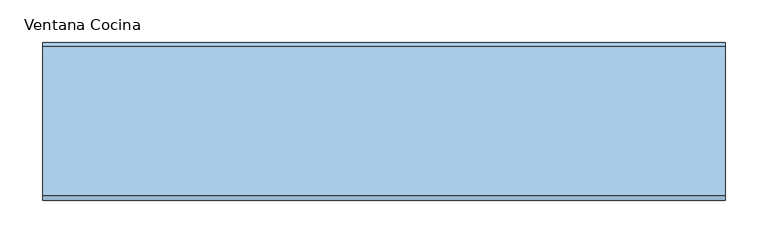
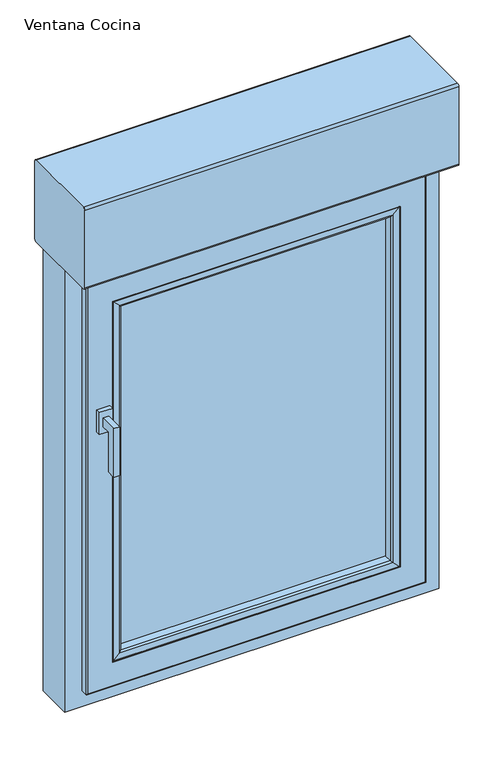
"""IFC4 building model written with IfcOpenShell, lengths in millimetres: window geometry, 2019_ES_Ventana_Replus_re80pvc301_10100_box_1-Hoja_con-Compacto : Ventana Cocina."""

from ifc_helpers import new_model, si_unit, point, frame, frame_2d, origin, place, context, project, spatial, polyline, circle_curve, ellipse_curve, trimmed, segment, composite_curve, outline, extrude, source, transform, mapped, element, save
from ifc_brep_helpers import plane_surface, cylinder_surface, advanced_brep


def ventana_cocina_c5497abf(model_context):
    return source(origin(), model_context, "Body", "SolidModel", [
        extrude(outline(composite_curve([segment(polyline([(55.0, 1810.0), (-120.0, 1810.0)]), True, "CONTINUOUS"), segment(trimmed(circle_curve(frame_2d((-120.0, 1815.0)), 5.0), [point((-120.0, 1810.0))], [point((-125.0, 1815.0))], False, "CARTESIAN"), True, "CONTINUOUS"), segment(polyline([(-125.0, 1815.0), (-125.0, 1990.0)]), True, "CONTINUOUS"), segment(trimmed(circle_curve(frame_2d((-120.0, 1990.0)), 5.0), [point((-125.0, 1990.0))], [point((-120.0, 1995.0))], False, "CARTESIAN"), True, "CONTINUOUS"), segment(polyline([(-120.0, 1995.0), (55.0, 1995.0)]), True, "CONTINUOUS"), segment(trimmed(circle_curve(frame_2d((55.0, 1990.0)), 5.0), [point((55.0, 1995.0))], [point((60.0, 1990.0))], False, "CARTESIAN"), True, "CONTINUOUS"), segment(polyline([(60.0, 1990.0), (60.0, 1815.0)]), True, "CONTINUOUS"), segment(trimmed(circle_curve(frame_2d((55.0, 1815.0)), 5.0), [point((60.0, 1815.0))], [point((55.0, 1810.0))], False, "CARTESIAN"), True, "CONTINUOUS")], self_intersect=False)), frame((-400.0, 0.0, 0.0), z_axis=(1.0, 0.0, 0.0), x_axis=(0.0, 1.0, 0.0)), (0.0, 0.0, 1.0), 800.0),
        extrude(outline(polyline([(-78.4999991, 1470.0), (-78.4999991, 1450.0), (-98.4999991, 1450.0), (-98.4999991, 1360.0), (-118.4999991, 1360.0), (-118.4999991, 1470.0), (-78.4999991, 1470.0)])), frame((-334.1999993, 0.0, 0.0), z_axis=(1.0, 0.0, 0.0), x_axis=(0.0, 1.0, 0.0)), (0.0, 0.0, 1.0), 12.0),
        extrude(outline(polyline([(-313.9687607, -78.4999991), (-342.4312378, -78.4999991), (-342.4312378, -68.4999991), (-313.9687607, -68.4999991), (-313.9687607, -78.4999991)])), frame((0.0, 0.0, 1435.217127), z_axis=(0.0, 0.0, 1.0), x_axis=(1.0, 0.0, 0.0)), (0.0, 0.0, 1.0), 49.565746),
        extrude(outline(polyline([(1707.2, 297.1999993), (1707.2, -297.1999993), (909.8, -297.1999993), (909.8, 297.1999993), (1707.2, 297.1999993)]), holes=[polyline([(917.8, 289.1999993), (917.8, -289.1999993), (1699.2, -289.1999993), (1699.2, 289.1999993), (917.8, 289.1999993)])]), frame((0.0, -26.9999999, 0.0), z_axis=(0.0, 1.0, 0.0), x_axis=(0.0, 0.0, 1.0)), (0.0, 0.0, 1.0), 16.0),
        extrude(outline(polyline([(1707.1868066, 297.1868058), (1707.1868066, -297.1868058), (909.8131934, -297.1868058), (909.8131934, 297.1868058), (1707.1868066, 297.1868058)]), holes=[polyline([(917.8, 289.1999993), (917.8, -289.1999993), (1699.2, -289.1999993), (1699.2, 289.1999993), (917.8, 289.1999993)])]), frame((0.0, -47.0000001, 0.0), z_axis=(0.0, 1.0, 0.0), x_axis=(0.0, 0.0, 1.0)), (0.0, 0.0, 1.0), 16.0),
        extrude(outline(polyline([(297.1999993, -6.9999997), (297.1999993, -10.9999999), (-297.1999993, -10.9999999), (-297.1999993, -6.9999997), (297.1999993, -6.9999997)])), frame((0.0, 0.0, 903.7946451), z_axis=(0.0, 0.0, 1.0), x_axis=(1.0, 0.0, 0.0)), (0.0, 0.0, 1.0), 809.4053549),
        extrude(outline(polyline([(297.1999993, -26.9999999), (297.1999993, -31.0000001), (-297.1999993, -31.0000001), (-297.1999993, -26.9999999), (297.1999993, -26.9999999)])), frame((0.0, 0.0, 903.7946451), z_axis=(0.0, 0.0, 1.0), x_axis=(1.0, 0.0, 0.0)), (0.0, 0.0, 1.0), 809.4053549),
        extrude(outline(polyline([(297.1999993, -47.0000001), (297.1999993, -51.0000003), (-297.1999993, -51.0000003), (-297.1999993, -47.0000001), (297.1999993, -47.0000001)])), frame((0.0, 0.0, 903.7946451), z_axis=(0.0, 0.0, 1.0), x_axis=(1.0, 0.0, 0.0)), (0.0, 0.0, 1.0), 809.4053549),
        advanced_brep(
        [(287.2913171, 9.2764571, 1697.2913178), (290.1890946, 11.5, 1700.1890953), (290.1890946, 11.5, 919.8109047), (287.2913171, 9.2764571, 922.7086822), (330.1999993, 11.5, 879.8), (-330.1999993, 11.5, 879.8), (-330.1999993, 11.5, 1740.2), (330.1999993, 11.5, 1740.2), (-290.1890946, 11.5, 1700.1890953), (-290.1890946, 11.5, 919.8109047), (-287.2913171, 9.2764571, 922.7086822), (284.1757968, -2.3508228, 1694.1757976), (284.1757968, -2.3508228, 925.8242024), (-284.1757968, -2.3508228, 925.8242024), (284.6739305, -3.0000033, 1694.6739313), (284.6739305, -3.0000033, 925.3260687), (-284.6739305, -3.0000033, 925.3260687), (291.1999993, -3.0000033, 1701.2), (-291.1999993, -3.0000033, 1701.2), (-291.1999993, -3.0000033, 918.8), (291.1999993, -3.0000033, 918.8), (-284.6739305, -3.0000033, 1694.6739313), (291.1999993, -6.9999997, 1701.2), (291.1999993, -6.9999997, 918.8), (-291.1999993, -6.9999997, 918.8), (311.8162192, -6.9999997, 1721.8162199), (-311.8162192, -6.9999997, 1721.8162199), (-311.8162192, -6.9999997, 898.1837801), (311.8162192, -6.9999997, 898.1837801), (-291.1999993, -6.9999997, 1701.2), (309.1999993, -25.6153717, 1719.2), (309.1999993, -25.6153717, 900.8), (-309.1999993, -25.6153717, 900.8), (309.1999993, -56.4999995, 1719.2), (309.1999993, -56.4999995, 900.8), (-309.1999993, -56.4999995, 900.8), (-309.1999993, -56.4999995, 1719.2), (297.1999993, -56.4999995, 1707.2), (-297.1999993, -56.4999995, 1707.2), (-297.1999993, -56.4999995, 912.8), (297.1999993, -56.4999995, 912.8), (297.1999993, -51.0000003, 1707.2), (297.1999993, -51.0000003, 912.8), (-297.1999993, -51.0000003, 912.8), (-297.1999993, -51.0000003, 1707.2), (286.007687, -51.0000003, 1696.0076877), (-286.007687, -51.0000003, 1696.0076877), (-286.007687, -51.0000003, 923.9923123), (286.007687, -51.0000003, 923.9923123), (285.4940999, -51.6693201, 1695.4941006), (285.4940999, -51.6693201, 924.5058994), (-285.4940999, -51.6693201, 924.5058994), (288.8993918, -64.3780426, 1698.8993925), (288.8993918, -64.3780426, 921.1006075), (-288.8993918, -64.3780426, 921.1006075), (292.6234971, -67.3403297, 1702.6234978), (292.6234971, -67.3403297, 917.3765022), (-292.6234971, -67.3403297, 917.3765022), (305.6488427, -67.7951848, 1715.6488434), (305.6488427, -67.7951848, 904.3511566), (-305.6488427, -67.7951848, 904.3511566), (306.1999993, -67.2629391, 1716.2), (306.1999993, -67.2629391, 903.8), (-306.1999993, -67.2629391, 903.8), (307.4370593, -68.4999991, 1717.43706), (307.4370593, -68.4999991, 902.56294), (-307.4370593, -68.4999991, 902.56294), (360.1999993, -68.4999991, 1770.2), (-360.1999993, -68.4999991, 1770.2), (-360.1999993, -68.4999991, 849.8), (360.1999993, -68.4999991, 849.8), (-307.4370593, -68.4999991, 1717.43706), (363.1999993, -65.4999991, 1773.2), (363.1999993, -65.4999991, 846.8), (-363.1999993, -65.4999991, 846.8), (363.1999993, -50.0, 1773.2), (363.1999993, -50.0, 846.8), (-363.1999993, -50.0, 846.8), (-363.1999993, -50.0, 1773.2), (343.1999993, -50.0, 1753.2), (-343.1999993, -50.0, 1753.2), (-343.1999993, -50.0, 866.8), (343.1999993, -50.0, 866.8), (343.1999993, -11.9999991, 866.8), (343.1999993, -11.9999991, 1753.2), (-343.1999993, -11.9999991, 866.8), (-343.1999993, -11.9999991, 1753.2), (330.1999993, -11.9999991, 1740.2), (-330.1999993, -11.9999991, 1740.2), (-330.1999993, -11.9999991, 879.8), (330.1999993, -11.9999991, 879.8), (-287.2913171, 9.2764571, 1697.2913178), (-284.1757968, -2.3508228, 1694.1757976), (-309.1999993, -25.6153717, 1719.2), (-285.4940999, -51.6693201, 1695.4941006), (-288.8993918, -64.3780426, 1698.8993925), (-292.6234971, -67.3403297, 1702.6234978), (-305.6488427, -67.7951848, 1715.6488434), (-306.1999993, -67.2629391, 1716.2), (-363.1999993, -65.4999991, 1773.2)],
        [
            (0, 1, ellipse_curve(frame((290.1890946, 8.5, 1700.1890953), z_axis=(0.7071067811865475, 0.0, -0.7071067811865475), x_axis=(0.7071067811865474, 0.0, 0.7071067811865476)), 4.2426407, 3.0)),
            (1, 2),
            (2, 3, ellipse_curve(frame((290.1890946, 8.5, 919.8109047), z_axis=(0.7071067811865475, 0.0, 0.7071067811865475), x_axis=(-0.7071067811865474, 0.0, 0.7071067811865476)), 4.2426407, 3.0)),
            (3, 0),
            (4, 5),
            (5, 6),
            (6, 7),
            (7, 4),
            (1, 8),
            (8, 9),
            (9, 2),
            (9, 10, ellipse_curve(frame((-290.1890946, 8.5, 919.8109047), z_axis=(0.7071067811865475, 0.0, -0.7071067811865475), x_axis=(0.7071067811865476, 0.0, 0.7071067811865474)), 4.2426407, 3.0)),
            (10, 3),
            (11, 0),
            (3, 12),
            (12, 11),
            (10, 13),
            (13, 12),
            (14, 11, ellipse_curve(frame((284.6739305, -2.4842973, 1694.6739313), z_axis=(0.7071067811865475, 0.0, -0.7071067811865475), x_axis=(0.7071067811865474, 0.0, 0.7071067811865476)), 0.7293184, 0.515706)),
            (12, 15, ellipse_curve(frame((284.6739305, -2.4842973, 925.3260687), z_axis=(0.7071067811865475, 0.0, 0.7071067811865475), x_axis=(-0.7071067811865474, 0.0, 0.7071067811865476)), 0.7293184, 0.515706)),
            (15, 14),
            (13, 16, ellipse_curve(frame((-284.6739305, -2.4842973, 925.3260687), z_axis=(0.7071067811865475, 0.0, -0.7071067811865475), x_axis=(0.7071067811865476, 0.0, 0.7071067811865474)), 0.7293184, 0.515706)),
            (16, 15),
            (17, 18),
            (18, 19),
            (19, 20),
            (20, 17),
            (16, 21),
            (21, 14),
            (22, 17),
            (20, 23),
            (23, 22),
            (19, 24),
            (24, 23),
            (25, 26),
            (26, 27),
            (27, 28),
            (28, 25),
            (24, 29),
            (29, 22),
            (30, 25),
            (28, 31),
            (31, 30),
            (27, 32),
            (32, 31),
            (33, 30),
            (31, 34),
            (34, 33),
            (32, 35),
            (35, 34),
            (35, 36),
            (36, 33),
            (37, 38),
            (38, 39),
            (39, 40),
            (40, 37),
            (41, 37),
            (40, 42),
            (42, 41),
            (39, 43),
            (43, 42),
            (43, 44),
            (44, 41),
            (45, 46),
            (46, 47),
            (47, 48),
            (48, 45),
            (49, 45, ellipse_curve(frame((286.007687, -51.5317048, 1696.0076877), z_axis=(0.7071067811865475, 0.0, -0.7071067811865475), x_axis=(0.7071067811865474, 0.0, 0.7071067811865476)), 0.7519437, 0.5317045)),
            (48, 50, ellipse_curve(frame((286.007687, -51.5317048, 923.9923123), z_axis=(0.7071067811865475, 0.0, 0.7071067811865475), x_axis=(-0.7071067811865474, 0.0, 0.7071067811865476)), 0.7519437, 0.5317045)),
            (50, 49),
            (47, 51, ellipse_curve(frame((-286.007687, -51.5317048, 923.9923123), z_axis=(0.7071067811865475, 0.0, -0.7071067811865475), x_axis=(0.7071067811865476, 0.0, 0.7071067811865474)), 0.7519437, 0.5317045)),
            (51, 50),
            (52, 49),
            (50, 53),
            (53, 52),
            (51, 54),
            (54, 53),
            (55, 52, ellipse_curve(frame((292.7630951, -63.3427664, 1702.7630958), z_axis=(0.7071067811865475, 0.0, -0.7071067811865475), x_axis=(0.7071067811865474, 0.0, 0.7071067811865476)), 5.6568542, 4.0)),
            (53, 56, ellipse_curve(frame((292.7630951, -63.3427664, 917.2369042), z_axis=(0.7071067811865475, 0.0, 0.7071067811865475), x_axis=(-0.7071067811865474, 0.0, 0.7071067811865476)), 5.6568542, 4.0)),
            (56, 55),
            (54, 57, ellipse_curve(frame((-292.7630951, -63.3427664, 917.2369042), z_axis=(0.7071067811865475, 0.0, -0.7071067811865475), x_axis=(0.7071067811865476, 0.0, 0.7071067811865474)), 5.6568542, 4.0)),
            (57, 56),
            (58, 55),
            (56, 59),
            (59, 58),
            (57, 60),
            (60, 59),
            (61, 58, ellipse_curve(frame((305.6674291, -67.2629391, 1715.6674299), z_axis=(0.7071067811865475, 0.0, -0.7071067811865475), x_axis=(0.7071067811865474, 0.0, 0.7071067811865476)), 0.7531679, 0.5325701)),
            (59, 62, ellipse_curve(frame((305.6674291, -67.2629391, 904.3325701), z_axis=(0.7071067811865475, 0.0, 0.7071067811865475), x_axis=(-0.7071067811865474, 0.0, 0.7071067811865476)), 0.7531679, 0.5325701)),
            (62, 61),
            (60, 63, ellipse_curve(frame((-305.6674291, -67.2629391, 904.3325701), z_axis=(0.7071067811865475, 0.0, -0.7071067811865475), x_axis=(0.7071067811865476, 0.0, 0.7071067811865474)), 0.7531679, 0.5325701)),
            (63, 62),
            (64, 61, ellipse_curve(frame((307.4370593, -67.2629391, 1717.43706), z_axis=(0.7071067811865475, 0.0, -0.7071067811865475), x_axis=(0.7071067811865474, 0.0, 0.7071067811865476)), 1.7494671, 1.23706)),
            (62, 65, ellipse_curve(frame((307.4370593, -67.2629391, 902.56294), z_axis=(0.7071067811865475, 0.0, 0.7071067811865475), x_axis=(-0.7071067811865474, 0.0, 0.7071067811865476)), 1.7494671, 1.23706)),
            (65, 64),
            (63, 66, ellipse_curve(frame((-307.4370593, -67.2629391, 902.56294), z_axis=(0.7071067811865475, 0.0, -0.7071067811865475), x_axis=(0.7071067811865476, 0.0, 0.7071067811865474)), 1.7494671, 1.23706)),
            (66, 65),
            (67, 68),
            (68, 69),
            (69, 70),
            (70, 67),
            (66, 71),
            (71, 64),
            (72, 67, ellipse_curve(frame((360.1999993, -65.4999991, 1770.2), z_axis=(0.7071067811865475, 0.0, -0.7071067811865475), x_axis=(0.7071067811865474, 0.0, 0.7071067811865476)), 4.2426407, 3.0)),
            (70, 73, ellipse_curve(frame((360.1999993, -65.4999991, 849.8), z_axis=(0.7071067811865475, 0.0, 0.7071067811865475), x_axis=(-0.7071067811865474, 0.0, 0.7071067811865476)), 4.2426407, 3.0)),
            (73, 72),
            (69, 74, ellipse_curve(frame((-360.1999993, -65.4999991, 849.8), z_axis=(0.7071067811865475, 0.0, -0.7071067811865475), x_axis=(0.7071067811865476, 0.0, 0.7071067811865474)), 4.2426407, 3.0)),
            (74, 73),
            (75, 72),
            (73, 76),
            (76, 75),
            (74, 77),
            (77, 76),
            (77, 78),
            (78, 75),
            (79, 80),
            (80, 81),
            (81, 82),
            (82, 79),
            (82, 83),
            (83, 84),
            (84, 79),
            (81, 85),
            (85, 83),
            (85, 86),
            (86, 84),
            (87, 88),
            (88, 89),
            (89, 90),
            (90, 87),
            (90, 4),
            (7, 87),
            (89, 5),
            (8, 91, ellipse_curve(frame((-290.1890946, 8.5, 1700.1890953), z_axis=(-0.7071067811865475, 0.0, -0.7071067811865475), x_axis=(0.7071067811865474, 0.0, -0.7071067811865476)), 4.2426407, 3.0)),
            (91, 10),
            (91, 92),
            (92, 13),
            (92, 21, ellipse_curve(frame((-284.6739305, -2.4842973, 1694.6739313), z_axis=(-0.7071067811865475, 0.0, -0.7071067811865475), x_axis=(0.7071067811865474, 0.0, -0.7071067811865476)), 0.7293184, 0.515706)),
            (18, 29),
            (26, 93),
            (93, 32),
            (93, 36),
            (38, 44),
            (46, 94, ellipse_curve(frame((-286.007687, -51.5317048, 1696.0076877), z_axis=(-0.7071067811865475, 0.0, -0.7071067811865475), x_axis=(0.7071067811865474, 0.0, -0.7071067811865476)), 0.7519437, 0.5317045)),
            (94, 51),
            (94, 95),
            (95, 54),
            (95, 96, ellipse_curve(frame((-292.7630951, -63.3427664, 1702.7630958), z_axis=(-0.7071067811865475, 0.0, -0.7071067811865475), x_axis=(0.7071067811865474, 0.0, -0.7071067811865476)), 5.6568542, 4.0)),
            (96, 57),
            (96, 97),
            (97, 60),
            (97, 98, ellipse_curve(frame((-305.6674291, -67.2629391, 1715.6674299), z_axis=(-0.7071067811865475, 0.0, -0.7071067811865475), x_axis=(0.7071067811865474, 0.0, -0.7071067811865476)), 0.7531679, 0.5325701)),
            (98, 63),
            (98, 71, ellipse_curve(frame((-307.4370593, -67.2629391, 1717.43706), z_axis=(-0.7071067811865475, 0.0, -0.7071067811865475), x_axis=(0.7071067811865474, 0.0, -0.7071067811865476)), 1.7494671, 1.23706)),
            (68, 99, ellipse_curve(frame((-360.1999993, -65.4999991, 1770.2), z_axis=(-0.7071067811865475, 0.0, -0.7071067811865475), x_axis=(0.7071067811865474, 0.0, -0.7071067811865476)), 4.2426407, 3.0)),
            (99, 74),
            (99, 78),
            (80, 86),
            (88, 6),
            (0, 91),
            (11, 92),
            (30, 93),
            (49, 94),
            (52, 95),
            (55, 96),
            (58, 97),
            (61, 98),
            (72, 99),
        ],
        [
            cylinder_surface(frame((290.1890946, 8.5, 1773.2), z_axis=(0.0, 0.0, 1.0), x_axis=(-1.0, 0.0, 0.0)), 3.0),
            plane_surface(frame((-330.1999993, 11.5, 1740.2), z_axis=(0.0, 1.0, 0.0), x_axis=(1.0, 0.0, 0.0))),
            cylinder_surface(frame((363.1999993, 8.5, 919.8109047), z_axis=(1.0, 0.0, 0.0), x_axis=(0.0, 0.0, 1.0)), 3.0),
            plane_surface(frame((287.2913171, 9.2764571, 1697.2913178), z_axis=(-0.9659258263570556, 0.258819044848789, 0.0), x_axis=(0.0, 0.0, -1.0))),
            plane_surface(frame((287.2913171, 9.2764571, 922.7086822), z_axis=(0.0, 0.2588190448487859, 0.9659258263570565), x_axis=(-1.0, 0.0, 0.0))),
            cylinder_surface(frame((284.6739305, -2.4842973, 1773.2), z_axis=(0.0, 0.0, 1.0), x_axis=(-1.0, 0.0, 0.0)), 0.515706),
            cylinder_surface(frame((363.1999993, -2.4842973, 925.3260687), z_axis=(1.0, 0.0, 0.0), x_axis=(0.0, 0.0, 1.0)), 0.515706),
            plane_surface(frame((-284.6739305, -3.0000033, 1694.6739313), z_axis=(0.0, -1.0, 0.0), x_axis=(1.0, 0.0, 0.0))),
            plane_surface(frame((291.1999993, -3.0000033, 1701.2), z_axis=(-1.0, 0.0, 0.0), x_axis=(0.0, 0.0, -1.0))),
            plane_surface(frame((291.1999993, -3.0000033, 918.8), z_axis=(0.0, 0.0, 1.0), x_axis=(-1.0, 0.0, 0.0))),
            plane_surface(frame((-291.1999993, -6.9999997, 1701.2), z_axis=(0.0, -1.0, 0.0), x_axis=(1.0, 0.0, 0.0))),
            plane_surface(frame((311.8162192, -6.9999997, 1721.8162199), z_axis=(-0.9902680687415736, 0.13917310096004265, 0.0), x_axis=(0.0, 0.0, -1.0))),
            plane_surface(frame((311.8162192, -6.9999997, 898.1837801), z_axis=(0.0, 0.13917310096003943, 0.990268068741574), x_axis=(-1.0, 0.0, 0.0))),
            plane_surface(frame((309.1999993, -25.6153717, 1719.2), z_axis=(-1.0, 0.0, 0.0), x_axis=(0.0, 0.0, -1.0))),
            plane_surface(frame((309.1999993, -25.6153717, 900.8), z_axis=(0.0, 0.0, 1.0), x_axis=(-1.0, 0.0, 0.0))),
            plane_surface(frame((-309.1999993, -56.4999995, 1719.2), z_axis=(0.0, 1.0, 0.0), x_axis=(1.0, 0.0, 0.0))),
            plane_surface(frame((297.1999993, -56.4999995, 1707.2), z_axis=(1.0, 0.0, 0.0), x_axis=(0.0, 0.0, -1.0))),
            plane_surface(frame((297.1999993, -56.4999995, 912.8), z_axis=(0.0, 0.0, -1.0), x_axis=(-1.0, 0.0, 0.0))),
            plane_surface(frame((-297.1999993, -51.0000003, 1707.2), z_axis=(0.0, 1.0, 0.0), x_axis=(1.0, 0.0, 0.0))),
            cylinder_surface(frame((286.007687, -51.5317048, 1773.2), z_axis=(0.0, 0.0, 1.0), x_axis=(-1.0, 0.0, 0.0)), 0.5317045),
            cylinder_surface(frame((363.1999993, -51.5317048, 923.9923123), z_axis=(1.0, 0.0, 0.0), x_axis=(0.0, 0.0, 1.0)), 0.5317045),
            plane_surface(frame((285.4940999, -51.6693201, 1695.4941006), z_axis=(-0.9659258262890666, -0.2588190451025272, 0.0), x_axis=(0.0, 0.0, -1.0))),
            plane_surface(frame((285.4940999, -51.6693201, 924.5058994), z_axis=(0.0, -0.2588190451025303, 0.9659258262890658), x_axis=(-1.0, 0.0, 0.0))),
            cylinder_surface(frame((292.7630951, -63.3427664, 1773.2), z_axis=(0.0, 0.0, 1.0), x_axis=(-1.0, 0.0, 0.0)), 4.0),
            cylinder_surface(frame((363.1999993, -63.3427664, 917.2369042), z_axis=(1.0, 0.0, 0.0), x_axis=(0.0, 0.0, 1.0)), 4.0),
            plane_surface(frame((292.6234971, -67.3403297, 1702.6234978), z_axis=(-0.03489949670250791, -0.9993908270190955, 0.0), x_axis=(0.0, 0.0, -1.0))),
            plane_surface(frame((292.6234971, -67.3403297, 917.3765022), z_axis=(0.0, -0.9993908270190957, 0.034899496702504675), x_axis=(-1.0, 0.0, 0.0))),
            cylinder_surface(frame((305.6674291, -67.2629391, 1773.2), z_axis=(0.0, 0.0, 1.0), x_axis=(-1.0, 0.0, 0.0)), 0.5325701),
            cylinder_surface(frame((363.1999993, -67.2629391, 904.3325701), z_axis=(1.0, 0.0, 0.0), x_axis=(0.0, 0.0, 1.0)), 0.5325701),
            cylinder_surface(frame((307.4370593, -67.2629391, 1773.2), z_axis=(0.0, 0.0, 1.0), x_axis=(-1.0, 0.0, 0.0)), 1.23706),
            cylinder_surface(frame((363.1999993, -67.2629391, 902.56294), z_axis=(1.0, 0.0, 0.0), x_axis=(0.0, 0.0, 1.0)), 1.23706),
            plane_surface(frame((-307.4370593, -68.4999991, 1717.43706), z_axis=(0.0, -1.0, 0.0), x_axis=(1.0, 0.0, 0.0))),
            cylinder_surface(frame((360.1999993, -65.4999991, 1773.2), z_axis=(0.0, 0.0, 1.0), x_axis=(-1.0, 0.0, 0.0)), 3.0),
            cylinder_surface(frame((363.1999993, -65.4999991, 849.8), z_axis=(1.0, 0.0, 0.0), x_axis=(0.0, 0.0, 1.0)), 3.0),
            plane_surface(frame((363.1999993, -65.4999991, 1773.2), z_axis=(1.0, 0.0, 0.0), x_axis=(0.0, 0.0, -1.0))),
            plane_surface(frame((363.1999993, -65.4999991, 846.8), z_axis=(0.0, 0.0, -1.0), x_axis=(-1.0, 0.0, 0.0))),
            plane_surface(frame((-359.2000019, -50.0, 1769.2000027), z_axis=(0.0, 1.0, 0.0), x_axis=(1.0, 0.0, 0.0))),
            plane_surface(frame((343.1999993, -45.0999991, 1753.2), z_axis=(1.0, 0.0, 0.0), x_axis=(0.0, 0.0, -1.0))),
            plane_surface(frame((343.1999993, -45.0999991, 866.8), z_axis=(0.0, 0.0, -1.0), x_axis=(-1.0, 0.0, 0.0))),
            plane_surface(frame((-335.7000002, -11.9999991, 1745.7000009), z_axis=(0.0, 1.0, 0.0), x_axis=(1.0, 0.0, 0.0))),
            plane_surface(frame((330.1999993, -1.4999991, 1740.2), z_axis=(1.0, 0.0, 0.0), x_axis=(0.0, 0.0, -1.0))),
            plane_surface(frame((330.1999993, -1.4999991, 879.8), z_axis=(0.0, 0.0, -1.0), x_axis=(-1.0, 0.0, 0.0))),
            cylinder_surface(frame((-290.1890946, 8.5, 846.8), z_axis=(0.0, 0.0, -1.0), x_axis=(1.0, 0.0, 0.0)), 3.0),
            plane_surface(frame((-287.2913171, 9.2764571, 922.7086822), z_axis=(0.9659258263570573, 0.25881904484878276, 0.0), x_axis=(0.0, 0.0, 1.0))),
            cylinder_surface(frame((-284.6739305, -2.4842973, 846.8), z_axis=(0.0, 0.0, -1.0), x_axis=(1.0, 0.0, 0.0)), 0.515706),
            plane_surface(frame((-291.1999993, -3.0000033, 918.8), z_axis=(1.0, 0.0, 0.0), x_axis=(0.0, 0.0, 1.0))),
            plane_surface(frame((-311.8162192, -6.9999997, 898.1837801), z_axis=(0.9902680687415745, 0.1391731009600362, 0.0), x_axis=(0.0, 0.0, 1.0))),
            plane_surface(frame((-309.1999993, -25.6153717, 900.8), z_axis=(1.0, 0.0, 0.0), x_axis=(0.0, 0.0, 1.0))),
            plane_surface(frame((-297.1999993, -56.4999995, 912.8), z_axis=(-1.0, 0.0, 0.0), x_axis=(0.0, 0.0, 1.0))),
            cylinder_surface(frame((-286.007687, -51.5317048, 846.8), z_axis=(0.0, 0.0, -1.0), x_axis=(1.0, 0.0, 0.0)), 0.5317045),
            plane_surface(frame((-285.4940999, -51.6693201, 924.5058994), z_axis=(0.9659258262890649, -0.2588190451025334, 0.0), x_axis=(0.0, 0.0, 1.0))),
            cylinder_surface(frame((-292.7630951, -63.3427664, 846.8), z_axis=(0.0, 0.0, -1.0), x_axis=(1.0, 0.0, 0.0)), 4.0),
            plane_surface(frame((-292.6234971, -67.3403297, 917.3765022), z_axis=(0.03489949670250144, -0.9993908270190958, 0.0), x_axis=(0.0, 0.0, 1.0))),
            cylinder_surface(frame((-305.6674291, -67.2629391, 846.8), z_axis=(0.0, 0.0, -1.0), x_axis=(1.0, 0.0, 0.0)), 0.5325701),
            cylinder_surface(frame((-307.4370593, -67.2629391, 846.8), z_axis=(0.0, 0.0, -1.0), x_axis=(1.0, 0.0, 0.0)), 1.23706),
            cylinder_surface(frame((-360.1999993, -65.4999991, 846.8), z_axis=(0.0, 0.0, -1.0), x_axis=(1.0, 0.0, 0.0)), 3.0),
            plane_surface(frame((-363.1999993, -65.4999991, 846.8), z_axis=(-1.0, 0.0, 0.0), x_axis=(0.0, 0.0, 1.0))),
            plane_surface(frame((-343.1999993, -45.0999991, 866.8), z_axis=(-1.0, 0.0, 0.0), x_axis=(0.0, 0.0, 1.0))),
            plane_surface(frame((-330.1999993, -1.4999991, 879.8), z_axis=(-1.0, 0.0, 0.0), x_axis=(0.0, 0.0, 1.0))),
            cylinder_surface(frame((-363.1999993, 8.5, 1700.1890953), z_axis=(-1.0, 0.0, 0.0), x_axis=(0.0, 0.0, -1.0)), 3.0),
            plane_surface(frame((-287.2913171, 9.2764571, 1697.2913178), z_axis=(0.0, 0.2588190448487859, -0.9659258263570564), x_axis=(1.0, 0.0, 0.0))),
            cylinder_surface(frame((-363.1999993, -2.4842973, 1694.6739313), z_axis=(-1.0, 0.0, 0.0), x_axis=(0.0, 0.0, -1.0)), 0.515706),
            plane_surface(frame((-291.1999993, -3.0000033, 1701.2), z_axis=(0.0, 0.0, -1.0), x_axis=(1.0, 0.0, 0.0))),
            plane_surface(frame((-311.8162192, -6.9999997, 1721.8162199), z_axis=(0.0, 0.13917310096003943, -0.990268068741574), x_axis=(1.0, 0.0, 0.0))),
            plane_surface(frame((-309.1999993, -25.6153717, 1719.2), z_axis=(0.0, 0.0, -1.0), x_axis=(1.0, 0.0, 0.0))),
            plane_surface(frame((-297.1999993, -56.4999995, 1707.2), z_axis=(0.0, 0.0, 1.0), x_axis=(1.0, 0.0, 0.0))),
            cylinder_surface(frame((-363.1999993, -51.5317048, 1696.0076877), z_axis=(-1.0, 0.0, 0.0), x_axis=(0.0, 0.0, -1.0)), 0.5317045),
            plane_surface(frame((-285.4940999, -51.6693201, 1695.4941006), z_axis=(0.0, -0.2588190451025303, -0.9659258262890658), x_axis=(1.0, 0.0, 0.0))),
            cylinder_surface(frame((-363.1999993, -63.3427664, 1702.7630958), z_axis=(-1.0, 0.0, 0.0), x_axis=(0.0, 0.0, -1.0)), 4.0),
            plane_surface(frame((-292.6234971, -67.3403297, 1702.6234978), z_axis=(0.0, -0.9993908270190957, -0.034899496702504675), x_axis=(1.0, 0.0, 0.0))),
            cylinder_surface(frame((-363.1999993, -67.2629391, 1715.6674299), z_axis=(-1.0, 0.0, 0.0), x_axis=(0.0, 0.0, -1.0)), 0.5325701),
            cylinder_surface(frame((-363.1999993, -67.2629391, 1717.43706), z_axis=(-1.0, 0.0, 0.0), x_axis=(0.0, 0.0, -1.0)), 1.23706),
            cylinder_surface(frame((-363.1999993, -65.4999991, 1770.2), z_axis=(-1.0, 0.0, 0.0), x_axis=(0.0, 0.0, -1.0)), 3.0),
            plane_surface(frame((-363.1999993, -65.4999991, 1773.2), z_axis=(0.0, 0.0, 1.0), x_axis=(1.0, 0.0, 0.0))),
            plane_surface(frame((-343.1999993, -45.0999991, 1753.2), z_axis=(0.0, 0.0, 1.0), x_axis=(1.0, 0.0, 0.0))),
            plane_surface(frame((-330.1999993, -1.4999991, 1740.2), z_axis=(0.0, 0.0, 1.0), x_axis=(1.0, 0.0, 0.0))),
        ],
        [
            (0, [[1, 2, 3, 4]]),
            (1, [[5, 6, 7, 8], [9, 10, 11, -2]]),
            (2, [[-3, -11, 12, 13]]),
            (3, [[14, -4, 15, 16]]),
            (4, [[-15, -13, 17, 18]]),
            (5, [[19, -16, 20, 21]]),
            (6, [[-20, -18, 22, 23]]),
            (7, [[24, 25, 26, 27], [-23, 28, 29, -21]]),
            (8, [[30, -27, 31, 32]]),
            (9, [[-31, -26, 33, 34]]),
            (10, [[35, 36, 37, 38], [-34, 39, 40, -32]]),
            (11, [[41, -38, 42, 43]]),
            (12, [[-42, -37, 44, 45]]),
            (13, [[46, -43, 47, 48]]),
            (14, [[-47, -45, 49, 50]]),
            (15, [[-50, 51, 52, -48], [53, 54, 55, 56]]),
            (16, [[57, -56, 58, 59]]),
            (17, [[-58, -55, 60, 61]]),
            (18, [[-61, 62, 63, -59], [64, 65, 66, 67]]),
            (19, [[68, -67, 69, 70]]),
            (20, [[-69, -66, 71, 72]]),
            (21, [[73, -70, 74, 75]]),
            (22, [[-74, -72, 76, 77]]),
            (23, [[78, -75, 79, 80]]),
            (24, [[-79, -77, 81, 82]]),
            (25, [[83, -80, 84, 85]]),
            (26, [[-84, -82, 86, 87]]),
            (27, [[88, -85, 89, 90]]),
            (28, [[-89, -87, 91, 92]]),
            (29, [[93, -90, 94, 95]]),
            (30, [[-94, -92, 96, 97]]),
            (31, [[98, 99, 100, 101], [-97, 102, 103, -95]]),
            (32, [[104, -101, 105, 106]]),
            (33, [[-105, -100, 107, 108]]),
            (34, [[109, -106, 110, 111]]),
            (35, [[-110, -108, 112, 113]]),
            (36, [[-113, 114, 115, -111], [116, 117, 118, 119]]),
            (37, [[-119, 120, 121, 122]]),
            (38, [[-120, -118, 123, 124]]),
            (39, [[-124, 125, 126, -121], [127, 128, 129, 130]]),
            (40, [[-130, 131, -8, 132]]),
            (41, [[-131, -129, 133, -5]]),
            (42, [[-12, -10, 134, 135]]),
            (43, [[-17, -135, 136, 137]]),
            (44, [[-22, -137, 138, -28]]),
            (45, [[-33, -25, 139, -39]]),
            (46, [[-44, -36, 140, 141]]),
            (47, [[-49, -141, 142, -51]]),
            (48, [[-60, -54, 143, -62]]),
            (49, [[-71, -65, 144, 145]]),
            (50, [[-76, -145, 146, 147]]),
            (51, [[-81, -147, 148, 149]]),
            (52, [[-86, -149, 150, 151]]),
            (53, [[-91, -151, 152, 153]]),
            (54, [[-96, -153, 154, -102]]),
            (55, [[-107, -99, 155, 156]]),
            (56, [[-112, -156, 157, -114]]),
            (57, [[-123, -117, 158, -125]]),
            (58, [[-133, -128, 159, -6]]),
            (59, [[-134, -9, -1, 160]]),
            (60, [[-136, -160, -14, 161]]),
            (61, [[-138, -161, -19, -29]]),
            (62, [[-139, -24, -30, -40]]),
            (63, [[-140, -35, -41, 162]]),
            (64, [[-142, -162, -46, -52]]),
            (65, [[-143, -53, -57, -63]]),
            (66, [[-144, -64, -68, 163]]),
            (67, [[-146, -163, -73, 164]]),
            (68, [[-148, -164, -78, 165]]),
            (69, [[-150, -165, -83, 166]]),
            (70, [[-152, -166, -88, 167]]),
            (71, [[-154, -167, -93, -103]]),
            (72, [[-155, -98, -104, 168]]),
            (73, [[-157, -168, -109, -115]]),
            (74, [[-158, -116, -122, -126]]),
            (75, [[-159, -127, -132, -7]]),
        ],
    ),
        advanced_brep(
        [(323.2673545, 12.758819, 1733.2673545), (327.2913185, 27.7764571, 1737.2913185), (327.2913185, 27.7764571, 882.7086815), (323.2673545, 12.758819, 886.7326455), (330.189096, 30.0, 1740.189096), (330.189096, 30.0, 879.810904), (-327.2913185, 27.7764571, 882.7086815), (-323.2673545, 12.758819, 886.7326455), (324.2332803, 11.5, 1734.2332803), (324.2332803, 11.5, 885.7667197), (400.0, 30.0, 1810.0), (400.0, -50.0, 1810.0), (400.0, -50.0, 810.0), (400.0, 30.0, 810.0), (-400.0, -50.0, 1810.0), (-400.0, -50.0, 810.0), (356.1999993, -50.0, 853.8000007), (-356.1999993, -50.0, 853.8000007), (-356.1999993, -50.0, 1766.1999993), (356.1999993, -50.0, 1766.1999993), (-400.0, 30.0, 810.0), (-400.0, 30.0, 1810.0), (-330.189096, 30.0, 1740.189096), (-330.189096, 30.0, 879.810904), (336.1891471, -8.0, 1746.1891471), (336.1891471, 11.5, 1746.1891471), (336.1891471, 11.5, 873.8108529), (336.1891471, -8.0, 873.8108529), (-336.1891471, 11.5, 1746.1891471), (-336.1891471, 11.5, 873.8108529), (-324.2332803, 11.5, 885.7667197), (-324.2332803, 11.5, 1734.2332803), (-336.1891471, -8.0, 873.8108529), (355.1999993, -8.0, 1765.1999993), (-355.1999993, -8.0, 1765.1999993), (-355.1999993, -8.0, 854.8000007), (355.1999993, -8.0, 854.8000007), (-336.1891471, -8.0, 1746.1891471), (355.1999993, -49.0, 1765.1999993), (355.1999993, -49.0, 854.8000007), (-355.1999993, -49.0, 854.8000007), (-327.2913185, 27.7764571, 1737.2913185), (-323.2673545, 12.758819, 1733.2673545), (-355.1999993, -49.0, 1765.1999993)],
        [
            (0, 1),
            (1, 2),
            (2, 3),
            (3, 0),
            (1, 4, ellipse_curve(frame((330.189096, 27.0, 1740.189096), z_axis=(0.7071067811865475, 0.0, -0.7071067811865475), x_axis=(0.7071067811865474, 0.0, 0.7071067811865476)), 4.2426407, 3.0)),
            (4, 5),
            (5, 2, ellipse_curve(frame((330.189096, 27.0, 879.810904), z_axis=(0.7071067811865475, 0.0, 0.7071067811865475), x_axis=(-0.7071067811865474, 0.0, 0.7071067811865476)), 4.2426407, 3.0)),
            (2, 6),
            (6, 7),
            (7, 3),
            (8, 0, ellipse_curve(frame((324.2332803, 12.5, 1734.2332803), z_axis=(0.7071067811865475, 0.0, -0.7071067811865475), x_axis=(0.7071067811865474, 0.0, 0.7071067811865476)), 1.4142136, 1.0)),
            (3, 9, ellipse_curve(frame((324.2332803, 12.5, 885.7667197), z_axis=(0.7071067811865475, 0.0, 0.7071067811865475), x_axis=(-0.7071067811865474, 0.0, 0.7071067811865476)), 1.4142136, 1.0)),
            (9, 8),
            (10, 11),
            (11, 12),
            (12, 13),
            (13, 10),
            (11, 14),
            (14, 15),
            (15, 12),
            (16, 17),
            (17, 18),
            (18, 19),
            (19, 16),
            (15, 20),
            (20, 13),
            (20, 21),
            (21, 10),
            (4, 22),
            (22, 23),
            (23, 5),
            (24, 25),
            (25, 26),
            (26, 27),
            (27, 24),
            (25, 28),
            (28, 29),
            (29, 26),
            (9, 30),
            (30, 31),
            (31, 8),
            (29, 32),
            (32, 27),
            (33, 34),
            (34, 35),
            (35, 36),
            (36, 33),
            (32, 37),
            (37, 24),
            (19, 38, ellipse_curve(frame((356.1999993, -49.0, 1766.1999993), z_axis=(0.7071067811865475, 0.0, -0.7071067811865475), x_axis=(0.7071067811865474, 0.0, 0.7071067811865476)), 1.4142136, 1.0)),
            (38, 39),
            (39, 16, ellipse_curve(frame((356.1999993, -49.0, 853.8000007), z_axis=(0.7071067811865475, 0.0, 0.7071067811865475), x_axis=(-0.7071067811865474, 0.0, 0.7071067811865476)), 1.4142136, 1.0)),
            (38, 33),
            (36, 39),
            (39, 40),
            (40, 17, ellipse_curve(frame((-356.1999993, -49.0, 853.8000007), z_axis=(0.7071067811865475, 0.0, -0.7071067811865475), x_axis=(0.7071067811865476, 0.0, 0.7071067811865474)), 1.4142136, 1.0)),
            (7, 30, ellipse_curve(frame((-324.2332803, 12.5, 885.7667197), z_axis=(0.7071067811865475, 0.0, -0.7071067811865475), x_axis=(0.7071067811865476, 0.0, 0.7071067811865474)), 1.4142136, 1.0)),
            (23, 6, ellipse_curve(frame((-330.189096, 27.0, 879.810904), z_axis=(0.7071067811865475, 0.0, -0.7071067811865475), x_axis=(0.7071067811865476, 0.0, 0.7071067811865474)), 4.2426407, 3.0)),
            (6, 41),
            (41, 42),
            (42, 7),
            (14, 21),
            (28, 37),
            (35, 40),
            (40, 43),
            (43, 18, ellipse_curve(frame((-356.1999993, -49.0, 1766.1999993), z_axis=(-0.7071067811865475, 0.0, -0.7071067811865475), x_axis=(0.7071067811865474, 0.0, -0.7071067811865476)), 1.4142136, 1.0)),
            (42, 31, ellipse_curve(frame((-324.2332803, 12.5, 1734.2332803), z_axis=(-0.7071067811865475, 0.0, -0.7071067811865475), x_axis=(0.7071067811865474, 0.0, -0.7071067811865476)), 1.4142136, 1.0)),
            (22, 41, ellipse_curve(frame((-330.189096, 27.0, 1740.189096), z_axis=(-0.7071067811865475, 0.0, -0.7071067811865475), x_axis=(0.7071067811865474, 0.0, -0.7071067811865476)), 4.2426407, 3.0)),
            (34, 43),
            (41, 1),
            (0, 42),
            (43, 38),
        ],
        [
            plane_surface(frame((327.2913185, 27.7764571, 1737.2913185), z_axis=(-0.9659258262890693, 0.25881904510251696, 0.0), x_axis=(0.0, 0.0, -1.0))),
            cylinder_surface(frame((330.189096, 27.0, 1810.0), z_axis=(0.0, 0.0, 1.0), x_axis=(-1.0, 0.0, 0.0)), 3.0),
            plane_surface(frame((327.2913185, 27.7764571, 882.7086815), z_axis=(0.0, 0.25881904510251386, 0.9659258262890702), x_axis=(-1.0, 0.0, 0.0))),
            cylinder_surface(frame((324.2332803, 12.5, 1810.0), z_axis=(0.0, 0.0, 1.0), x_axis=(-1.0, 0.0, 0.0)), 1.0),
            plane_surface(frame((400.0, -50.0, 1810.0), z_axis=(1.0, 0.0, 0.0), x_axis=(0.0, 0.0, -1.0))),
            plane_surface(frame((-356.1999993, -50.0, 1766.1999993), z_axis=(0.0, -1.0, 0.0), x_axis=(1.0, 0.0, 0.0))),
            plane_surface(frame((400.0, -50.0, 810.0), z_axis=(0.0, 0.0, -1.0), x_axis=(-1.0, 0.0, 0.0))),
            plane_surface(frame((-400.0, 30.0, 1810.0), z_axis=(0.0, 1.0, 0.0), x_axis=(1.0, 0.0, 0.0))),
            plane_surface(frame((336.1891471, 11.5, 1746.1891471), z_axis=(-1.0, 0.0, 0.0), x_axis=(0.0, 0.0, -1.0))),
            plane_surface(frame((-324.2332803, 11.5, 1734.2332803), z_axis=(0.0, -1.0, 0.0), x_axis=(1.0, 0.0, 0.0))),
            plane_surface(frame((336.1891471, 11.5, 873.8108529), z_axis=(0.0, 0.0, 1.0), x_axis=(-1.0, 0.0, 0.0))),
            plane_surface(frame((-336.1891471, -8.0, 1746.1891471), z_axis=(0.0, -1.0, 0.0), x_axis=(1.0, 0.0, 0.0))),
            cylinder_surface(frame((356.1999993, -49.0, 1810.0), z_axis=(0.0, 0.0, 1.0), x_axis=(-1.0, 0.0, 0.0)), 1.0),
            plane_surface(frame((355.1999993, -8.0, 1765.1999993), z_axis=(-1.0, 0.0, 0.0), x_axis=(0.0, 0.0, -1.0))),
            cylinder_surface(frame((400.0, -49.0, 853.8000007), z_axis=(1.0, 0.0, 0.0), x_axis=(0.0, 0.0, 1.0)), 1.0),
            cylinder_surface(frame((400.0, 12.5, 885.7667197), z_axis=(1.0, 0.0, 0.0), x_axis=(0.0, 0.0, 1.0)), 1.0),
            cylinder_surface(frame((400.0, 27.0, 879.810904), z_axis=(1.0, 0.0, 0.0), x_axis=(0.0, 0.0, 1.0)), 3.0),
            plane_surface(frame((-327.2913185, 27.7764571, 882.7086815), z_axis=(0.9659258262890711, 0.25881904510251075, 0.0), x_axis=(0.0, 0.0, 1.0))),
            plane_surface(frame((-400.0, -50.0, 810.0), z_axis=(-1.0, 0.0, 0.0), x_axis=(0.0, 0.0, 1.0))),
            plane_surface(frame((-336.1891471, 11.5, 873.8108529), z_axis=(1.0, 0.0, 0.0), x_axis=(0.0, 0.0, 1.0))),
            plane_surface(frame((355.1999993, -8.0, 854.8000007), z_axis=(0.0, 0.0, 1.0), x_axis=(-1.0, 0.0, 0.0))),
            cylinder_surface(frame((-356.1999993, -49.0, 810.0), z_axis=(0.0, 0.0, -1.0), x_axis=(1.0, 0.0, 0.0)), 1.0),
            cylinder_surface(frame((-324.2332803, 12.5, 810.0), z_axis=(0.0, 0.0, -1.0), x_axis=(1.0, 0.0, 0.0)), 1.0),
            cylinder_surface(frame((-330.189096, 27.0, 810.0), z_axis=(0.0, 0.0, -1.0), x_axis=(1.0, 0.0, 0.0)), 3.0),
            plane_surface(frame((-355.1999993, -8.0, 854.8000007), z_axis=(1.0, 0.0, 0.0), x_axis=(0.0, 0.0, 1.0))),
            plane_surface(frame((-327.2913185, 27.7764571, 1737.2913185), z_axis=(0.0, 0.25881904510251386, -0.9659258262890702), x_axis=(1.0, 0.0, 0.0))),
            plane_surface(frame((-400.0, -50.0, 1810.0), z_axis=(0.0, 0.0, 1.0), x_axis=(1.0, 0.0, 0.0))),
            plane_surface(frame((-336.1891471, 11.5, 1746.1891471), z_axis=(0.0, 0.0, -1.0), x_axis=(1.0, 0.0, 0.0))),
            cylinder_surface(frame((-400.0, -49.0, 1766.1999993), z_axis=(-1.0, 0.0, 0.0), x_axis=(0.0, 0.0, -1.0)), 1.0),
            cylinder_surface(frame((-400.0, 12.5, 1734.2332803), z_axis=(-1.0, 0.0, 0.0), x_axis=(0.0, 0.0, -1.0)), 1.0),
            cylinder_surface(frame((-400.0, 27.0, 1740.189096), z_axis=(-1.0, 0.0, 0.0), x_axis=(0.0, 0.0, -1.0)), 3.0),
            plane_surface(frame((-355.1999993, -8.0, 1765.1999993), z_axis=(0.0, 0.0, -1.0), x_axis=(1.0, 0.0, 0.0))),
        ],
        [
            (0, [[1, 2, 3, 4]]),
            (1, [[5, 6, 7, -2]]),
            (2, [[-3, 8, 9, 10]]),
            (3, [[11, -4, 12, 13]]),
            (4, [[14, 15, 16, 17]]),
            (5, [[18, 19, 20, -15], [21, 22, 23, 24]]),
            (6, [[-16, -20, 25, 26]]),
            (7, [[-26, 27, 28, -17], [29, 30, 31, -6]]),
            (8, [[32, 33, 34, 35]]),
            (9, [[36, 37, 38, -33], [39, 40, 41, -13]]),
            (10, [[-34, -38, 42, 43]]),
            (11, [[44, 45, 46, 47], [-43, 48, 49, -35]]),
            (12, [[50, 51, 52, -24]]),
            (13, [[53, -47, 54, -51]]),
            (14, [[-52, 55, 56, -21]]),
            (15, [[-12, -10, 57, -39]]),
            (16, [[-7, -31, 58, -8]]),
            (17, [[-9, 59, 60, 61]]),
            (18, [[-25, -19, 62, -27]]),
            (19, [[-42, -37, 63, -48]]),
            (20, [[-54, -46, 64, -55]]),
            (21, [[-56, 65, 66, -22]]),
            (22, [[-57, -61, 67, -40]]),
            (23, [[-58, -30, 68, -59]]),
            (24, [[-64, -45, 69, -65]]),
            (25, [[-60, 70, -1, 71]]),
            (26, [[-62, -18, -14, -28]]),
            (27, [[-63, -36, -32, -49]]),
            (28, [[-66, 72, -50, -23]]),
            (29, [[-67, -71, -11, -41]]),
            (30, [[-68, -29, -5, -70]]),
            (31, [[-69, -44, -53, -72]]),
        ],
    ),
    ])


if __name__ == "__main__":
    model = new_model("IFC4")
    model_context = context("Model", 3, world=origin())
    ifc_project = project(units=[si_unit("LENGTHUNIT", "METRE", prefix="MILLI")], contexts=[model_context])
    site = spatial("IfcSite", under=ifc_project)
    building = spatial("IfcBuilding", under=site)
    placement = place(None, origin())
    ventana_cocina_shape = ventana_cocina_c5497abf(model_context)
    element("IfcWindow", 1, ObjectType="2019_ES_Ventana_Replus_re80pvc301_10100_box_1-Hoja_con-Compacto : Ventana Cocina", at=placement, inside=building, context=model_context, shape_type="MappedRepresentation", body=[
        mapped(ventana_cocina_shape, transform((0.0, 0.0, 0.0), x_axis=(1.0, 0.0, 0.0), y_axis=(0.0, 1.0, 0.0), z_axis=(0.0, 0.0, 1.0))),
    ])
    save(model, "model.ifc")

# Revit data of these elements
# Type "2019_ES_Ventana_Replus_re80pvc301_10100_box_1-Hoja_con-Compacto : Ventana Cocina"
#   Type Mark = "41"
#   URL = "https://replus.es/"
#   Product data url = "https://bimetica.com/es/objetos-bim-replus-ventana-practicable-oscilobatiente-una-hoja-con-compacto-9540"
#   Product Guid = ""
#   Model = "10100 BOX"
#   Material secondary = "Glass"
#   Material main = "PVC"
#   Manufacturer = "Replus"
#   Keynote = "08500"
#   EAN code = ""
#   Description = "Perfiles de PVC con triple junta (por junta rígida en el marco). Protegiendo de este modo todos los puntos de cierre y proporcionando una junta perimetral completa, con un grosor en el perfil de 3 mm. Vidrio de alta calidad con diferentes posibilidades"
#   Assembly Code = "B2020100"
#   Analytic Construction = "<None>"
#   Ι_Wll Thcknss [instance default] = 20.0 cm
#   Ι_Wdth Cntrl = 80.0 cm
#   Ι_Nst Cntrl [instance default] = 0.0 cm
#   Ι_Hndl Hght Cntrl = 65.0 cm
#   Ι_Hght Cntrl = 100.0 cm
#   Rough Width = 82.0 cm
#   Rough Height = 102.0 cm
#   Retranqueo [instance default] = 0.0 cm
#   I_Lf_Cntrl = 72.64 cm
#   Hueco = 1.0 cm
#   Height = 100.0 cm
#   Default Sill Height = 80.0 cm
#   Width = 80.0 cm
#   Altura de Manilla = 65.0 cm
#   Visibilidad Líneas Apertura - Planta = yes
#   Visibilidad Líneas Apertura - Alzado = yes
#   Exceso Dimensiones = no
#   Edition number = 1
#   Advertencia Dimensión = yes
#   Product Material = PVC - Replus - 9152 - White
#   Wall Closure = (empty or 0)
# Element 1 (IfcWindow, "2019_ES_Ventana_Replus_re80pvc301_10100_box_1-Hoja_con-Compacto : Ventana Cocina")
#   Ι_Wll Thcknss = 10.0 cm
#   Materials on its faces: "PVC - Replus - 9152 - White", "Rubber - Replus - Black", "Glass - Replus"
# Materials
#   "PVC - Replus - 9152 - White": class "Miscellaneous", colour RGB 174 174 166, transparency 0, Manufacturer = "Replus", Comments = "Rendering appearance not upgraded ", URL = "https://replus.es/", Cost = 0
#   "Rubber - Replus - Black": class "Plastic", colour RGB 63 63 63, transparency 0, Description = "Natural rubber, black", Cost = 0
#   "Glass - Replus": class "Glass", colour RGB 218 227 224, transparency 0.85, Cost = 0
